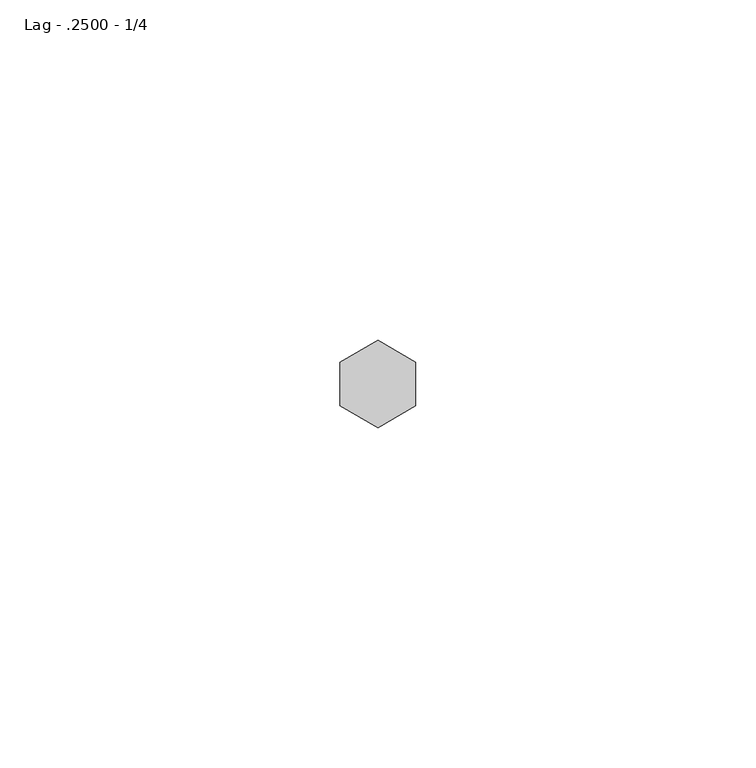
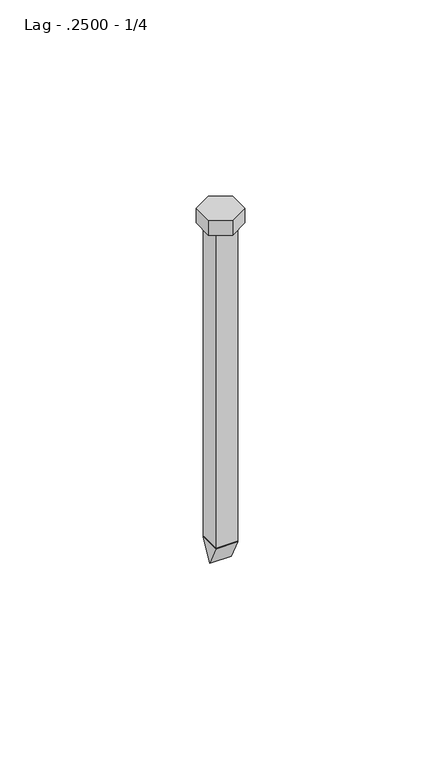
"""IFC4 building model written with IfcOpenShell, lengths in millimetres: fastener geometry, 060523 - W_P_C - Fastenings - Generic - SQUARE : Lag - .2500 - 1/4."""

import ifcopenshell
import ifcopenshell.guid

model = None  # the IFC model being written
_history = None  # IfcOwnerHistory: only IFC2X3 demands one
_inside = {}  # id of a spatial element -> (the spatial element, [elements in it])
_under = {}  # id of a project, library or spatial element -> (it, [spatial elements below it])
_declared = {}  # id of a project -> (the project, [libraries it declares])
_typed = {}  # id of a type object -> (the type object, [elements of that type])
_made_of = {}  # id of a material, layer set ... -> (it, [elements and type objects made of it])


def new_model(schema):
    """Start an empty IFC model of exactly this schema.

    Asked for "IFC4X3", IfcOpenShell would pick the latest addendum, in which some entities
    have other attributes; the version numbers below select the first issue.
    IFC2X3 requires an IfcOwnerHistory on every rooted entity: one is made here for all.
    """
    global model, _history
    if schema == "IFC4X3":
        model = ifcopenshell.file(schema_version=(4, 3, 0, 0))
    else:
        model = ifcopenshell.file(schema=schema)
    _inside.clear()
    _under.clear()
    _declared.clear()
    _typed.clear()
    _made_of.clear()
    _history = None
    if model.schema == "IFC2X3":
        org = make("IfcOrganization", Name="unknown")
        user = make(
            "IfcPersonAndOrganization",
            ThePerson=make("IfcPerson", FamilyName="unknown"),
            TheOrganization=org,
        )
        app = make(
            "IfcApplication",
            ApplicationDeveloper=org,
            Version="unknown",
            ApplicationFullName="unknown",
            ApplicationIdentifier="unknown",
        )
        _history = make(
            "IfcOwnerHistory",
            OwningUser=user,
            OwningApplication=app,
            ChangeAction="ADDED",
            CreationDate=0,
        )
    return model


def make(cls, **values):
    """One entity of the class cls with the attributes given. An attribute that is None is left unset."""
    return model.create_entity(
        cls, **{name: value for name, value in values.items() if value is not None}
    )


def rooted(cls, **values):
    """An entity with a GlobalId (a new one), such as an element, a storey or a relation."""
    return make(cls, GlobalId=ifcopenshell.guid.new(), OwnerHistory=_history, **values)


def si_unit(unit_type, name, prefix=None):
    """IfcSIUnit, for example si_unit("LENGTHUNIT", "METRE", prefix="MILLI")."""
    return make("IfcSIUnit", UnitType=unit_type, Prefix=prefix, Name=name)


def assignment(units):
    """IfcUnitAssignment: the units of a project."""
    return None if units is None else make("IfcUnitAssignment", Units=units)


def point(xyz):
    """IfcCartesianPoint."""
    return None if xyz is None else make("IfcCartesianPoint", Coordinates=xyz)


def direction(xyz):
    """IfcDirection."""
    return None if xyz is None else make("IfcDirection", DirectionRatios=xyz)


def frame(location, z_axis=None, x_axis=None):
    """IfcAxis2Placement3D, a coordinate frame: its origin and axes. An axis left out is left unset."""
    return make(
        "IfcAxis2Placement3D",
        Location=point(location),
        Axis=direction(z_axis),
        RefDirection=direction(x_axis),
    )


def origin():
    """The frame at (0, 0, 0) with its axes left unset."""
    return frame((0.0, 0.0, 0.0))


def origin_with_axes():
    """The frame at (0, 0, 0) with the z axis (0, 0, 1) and the x axis (1, 0, 0) written out."""
    return frame((0.0, 0.0, 0.0), z_axis=(0.0, 0.0, 1.0), x_axis=(1.0, 0.0, 0.0))


def place(relative_to, where):
    """IfcLocalPlacement: puts the frame where relative to a parent placement (None: the world)."""
    return make(
        "IfcLocalPlacement", PlacementRelTo=relative_to, RelativePlacement=where
    )


def context(
    kind, dimensions, precision=None, world=None, true_north=None, identifier=None
):
    """IfcGeometricRepresentationContext, for example the 3D "Model" context."""
    return make(
        "IfcGeometricRepresentationContext",
        ContextIdentifier=identifier,
        ContextType=kind,
        CoordinateSpaceDimension=dimensions,
        Precision=precision,
        WorldCoordinateSystem=world,
        TrueNorth=true_north,
    )


def project(units=None, contexts=None):
    """IfcProject with its units and contexts."""
    return rooted(
        "IfcProject",
        Name="project",
        RepresentationContexts=contexts,
        UnitsInContext=assignment(units),
    )


def spatial(cls, under=None, at=None, **own):
    """A site, building, storey or space (cls), placed at a placement, below another one or the project."""
    s = rooted(cls, ObjectPlacement=at, **own)
    if under is not None:
        _under.setdefault(under.id(), (under, []))[1].append(s)
    return s


def polyline(points):
    """IfcPolyline through the points."""
    return make("IfcPolyline", Points=[point(p) for p in points])


def outline(outer, holes=None, kind="AREA"):
    """IfcArbitraryClosedProfileDef: a profile drawn as a closed curve; with holes, ...WithVoids."""
    if holes is None:
        return make("IfcArbitraryClosedProfileDef", ProfileType=kind, OuterCurve=outer)
    return make(
        "IfcArbitraryProfileDefWithVoids",
        ProfileType=kind,
        OuterCurve=outer,
        InnerCurves=holes,
    )


def extrude(swept, where, along, depth):
    """IfcExtrudedAreaSolid: the profile swept, set in the frame where, extruded along a direction by depth."""
    return make(
        "IfcExtrudedAreaSolid",
        SweptArea=swept,
        Position=where,
        ExtrudedDirection=direction(along),
        Depth=depth,
    )


def shape(context_of_items, identifier, shape_type, items):
    """IfcShapeRepresentation: the items that make up one representation, for example the "Body"."""
    return make(
        "IfcShapeRepresentation",
        ContextOfItems=context_of_items,
        RepresentationIdentifier=identifier,
        RepresentationType=shape_type,
        Items=items,
    )


def source(mapping_origin, context_of_items, identifier, shape_type, items):
    """IfcRepresentationMap: a shape defined once, which mapped items show again and again."""
    return make(
        "IfcRepresentationMap",
        MappingOrigin=mapping_origin,
        MappedRepresentation=shape(context_of_items, identifier, shape_type, items),
    )


def transform(
    local_origin,
    x_axis=None,
    y_axis=None,
    z_axis=None,
    scale=None,
    scale2=None,
    scale3=None,
    uniform=True,
):
    """IfcCartesianTransformationOperator3D, or its non-uniform kind. x_axis, y_axis, z_axis: its Axis1, 2, 3."""
    if uniform:
        return make(
            "IfcCartesianTransformationOperator3D",
            Axis1=direction(x_axis),
            Axis2=direction(y_axis),
            LocalOrigin=point(local_origin),
            Scale=scale,
            Axis3=direction(z_axis),
        )
    return make(
        "IfcCartesianTransformationOperator3DnonUniform",
        Axis1=direction(x_axis),
        Axis2=direction(y_axis),
        LocalOrigin=point(local_origin),
        Scale=scale,
        Axis3=direction(z_axis),
        Scale2=scale2,
        Scale3=scale3,
    )


def mapped(mapping_source, mapping_target):
    """IfcMappedItem: shows the shape of a source again, moved by a transform."""
    return make(
        "IfcMappedItem", MappingSource=mapping_source, MappingTarget=mapping_target
    )


def made_of(thing, what):
    """Note that an element or type object is made of a material, layer set ...; save() writes the relation."""
    if what is not None:
        _made_of.setdefault(what.id(), (what, []))[1].append(thing)
    return thing


def element(
    cls,
    number,
    at=None,
    inside=None,
    cuts=None,
    type_object=None,
    material=None,
    context=None,
    identifier="Body",
    shape_type=None,
    held_by="IfcProductDefinitionShape",
    body=None,
    shapes=None,
    **own,
):
    """One element of the class cls, such as IfcWall. Its Tag is "e" and its number.

    at: its placement. inside: the storey or other place that contains it. cuts: it is an
    opening in that element (IfcRelVoidsElement). A single representation is given by context,
    identifier, shape_type and body (its items); several are given by shapes. held_by: the class
    of the entity that holds the representations. save() writes the other relations.
    """
    e = rooted(cls, Tag="e%d" % number, ObjectPlacement=at, **own)
    if body is not None:
        shapes = [shape(context, identifier, shape_type, body)]
    if shapes is not None:
        e.Representation = make(held_by, Representations=shapes)
    if inside is not None:
        _inside.setdefault(inside.id(), (inside, []))[1].append(e)
    if cuts is not None:
        rooted(
            "IfcRelVoidsElement", RelatingBuildingElement=cuts, RelatedOpeningElement=e
        )
    if type_object is not None:
        _typed.setdefault(type_object.id(), (type_object, []))[1].append(e)
    return made_of(e, material)


def aggregate(whole, parts):
    """IfcRelAggregates: a whole, such as a stair, and the parts it consists of."""
    return rooted("IfcRelAggregates", RelatingObject=whole, RelatedObjects=parts)


def save(model, path):
    """Write the relations noted so far, then the file.

    IfcRelAggregates (storeys below a building ...), IfcRelContainedInSpatialStructure (elements
    in a storey), IfcRelDefinesByType, IfcRelAssociatesMaterial and IfcRelDeclares: one each for
    every whole, place, type object, material and project.
    """
    for whole, parts in _under.values():
        aggregate(whole, parts)
    for where, things in _inside.values():
        rooted(
            "IfcRelContainedInSpatialStructure",
            RelatedElements=things,
            RelatingStructure=where,
        )
    for kind, things in _typed.values():
        rooted("IfcRelDefinesByType", RelatedObjects=things, RelatingType=kind)
    for what, things in _made_of.values():
        rooted("IfcRelAssociatesMaterial", RelatedObjects=things, RelatingMaterial=what)
    for by, libraries in _declared.values():
        rooted("IfcRelDeclares", RelatingContext=by, RelatedDefinitions=libraries)
    model.write(path)


def lag_2500_1_4_1fa157ba(model_context):
    return source(origin(), model_context, "Body", "SweptSolid", [
        extrude(outline(polyline([(0.0, -108.204), (-3.302, -101.6), (3.302, -101.6), (0.0, -108.204)])), frame((-3.302, 0.0, 0.0), z_axis=(1.0, 0.0, 0.0), x_axis=(0.0, 1.0, 0.0)), (0.0, 0.0, 1.0), 6.604),
        extrude(outline(polyline([(-5.55625, 3.2079024), (0.0, 6.4158049), (5.55625, 3.2079024), (5.55625, -3.2079024), (0.0, -6.4158049), (-5.55625, -3.2079024), (-5.55625, 3.2079024)])), origin_with_axes(), (0.0, 0.0, 1.0), 4.7625),
        extrude(outline(polyline([(-3.302, 3.302), (3.302, 3.302), (3.302, -3.302), (-3.302, -3.302), (-3.302, 3.302)])), frame((0.0, 0.0, -101.6), z_axis=(0.0, 0.0, 1.0), x_axis=(1.0, 0.0, 0.0)), (0.0, 0.0, 1.0), 101.6),
    ])


if __name__ == "__main__":
    model = new_model("IFC4")
    model_context = context("Model", 3, world=origin())
    ifc_project = project(units=[si_unit("LENGTHUNIT", "METRE", prefix="MILLI")], contexts=[model_context])
    site = spatial("IfcSite", under=ifc_project)
    building = spatial("IfcBuilding", under=site)
    placement = place(None, origin())
    lag_2500_1_4_shape = lag_2500_1_4_1fa157ba(model_context)
    element("IfcFastener", 1, ObjectType="060523 - W_P_C - Fastenings - Generic - SQUARE : Lag - .2500 - 1/4", at=placement, inside=building, context=model_context, shape_type="MappedRepresentation", body=[
        mapped(lag_2500_1_4_shape, transform((0.0, 0.0, 0.0), x_axis=(1.0, 0.0, 0.0), y_axis=(0.0, 1.0, 0.0), z_axis=(0.0, 0.0, 1.0))),
    ])
    save(model, "model.ifc")

# Revit data of these elements
# Type "060523 - W_P_C - Fastenings - Generic - SQUARE : Lag - .2500 - 1/4"
#   Washer_Thickness = 0' - 0 1/16"
#   Washer Radius = 0' - 0.3175"
#   Washer Offset - Head = 0' - 0"
#   Washer Offset = 0' - 0"
#   Thickness_of_Substrate [instance default] = 0' - 1"
#   Side = 0' - 0.25293"
#   Radius = 0' - 0.13"
#   Length [instance default] = 0' - 4"
#   Head Size = 0' - 0 7/16"
#   Head Radius = 0' - 0 7/32"
#   Head Height = 0' - 0 3/16"
#   Double Diameter = 0' - 0.52"
#   Diameter = 0' - 0.26"
#   Default Elevation = 4' - 0"
#   Washer_Nut_Visibility = no
#   Washer_Head_Visibility = no
#   Round_Head_Visibility = no
#   Point Visibility = yes
#   Nut_Visibility = no
#   Hex_Head_Visiblilty = yes
#   Washer Material = none
#   Bolt Material (Size) = AT SILL - FASTENER AT 24" O.C.
# Element 1 (IfcFastener, "060523 - W_P_C - Fastenings - Generic - SQUARE : Lag - .2500 - 1/4")
#   Materials on its faces: "AT SILL - FASTENER AT 24\" O.C."
# Materials
#   "AT SILL - FASTENER AT 24\" O.C.": class "Generic", colour RGB 120 120 120, transparency 0, Cost = 0
